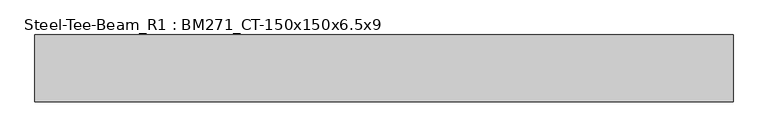
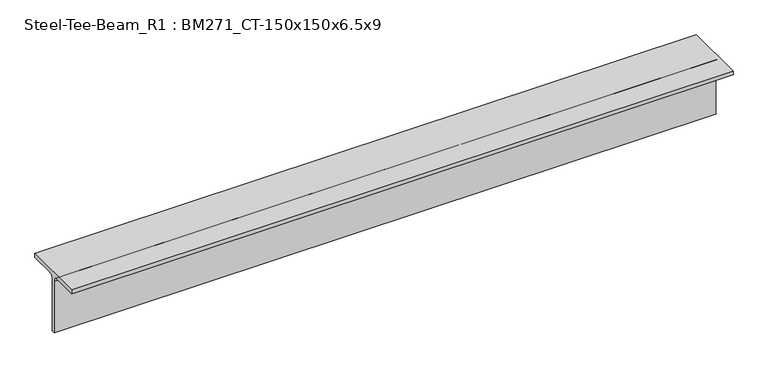
"""IFC4 building model written with IfcOpenShell, lengths in millimetres: member geometry, Steel-Tee-Beam_R1 : BM271_CT-150x150x6.5x9."""

from ifc_helpers import new_model, si_unit, point, frame, frame_2d, origin, place, context, project, spatial, polyline, circle_curve, trimmed, segment, composite_curve, outline, extrude, source, transform, mapped, element, save


def steel_tee_beam_r1_bm271_ct_150x150x6_5x9_cc699060(model_context):
    return source(origin(), model_context, "Body", "SweptSolid", [
        extrude(outline(composite_curve([segment(polyline([(-75.0, 75.0), (75.0, 75.0), (75.0, 66.0), (16.25, 66.0)]), True, "CONTINUOUS"), segment(trimmed(circle_curve(frame_2d((16.25, 53.0)), 13.0), [point((16.25, 66.0))], [point((3.25, 53.0))], True, "CARTESIAN"), True, "CONTINUOUS"), segment(polyline([(3.25, 53.0), (3.25, -75.0), (-3.25, -75.0), (-3.25, 53.0)]), True, "CONTINUOUS"), segment(trimmed(circle_curve(frame_2d((-16.25, 53.0)), 13.0), [point((-3.25, 53.0))], [point((-16.25, 66.0))], True, "CARTESIAN"), True, "CONTINUOUS"), segment(polyline([(-16.25, 66.0), (-75.0, 66.0), (-75.0, 75.0)]), True, "CONTINUOUS")], self_intersect=False)), frame((-860.2325267, 0.0, 0.0), z_axis=(1.0, 0.0, 0.0), x_axis=(0.0, 1.0, 0.0)), (0.0, 0.0, 1.0), 1562.0258541),
    ])


if __name__ == "__main__":
    model = new_model("IFC4")
    model_context = context("Model", 3, world=origin())
    ifc_project = project(units=[si_unit("LENGTHUNIT", "METRE", prefix="MILLI")], contexts=[model_context])
    site = spatial("IfcSite", under=ifc_project)
    building = spatial("IfcBuilding", under=site)
    placement = place(None, origin())
    steel_tee_beam_r1_bm271_ct_150x150x6_5x9_shape = steel_tee_beam_r1_bm271_ct_150x150x6_5x9_cc699060(model_context)
    element("IfcMember", 1, ObjectType="Steel-Tee-Beam_R1 : BM271_CT-150x150x6.5x9", at=placement, inside=building, context=model_context, shape_type="MappedRepresentation", body=[
        mapped(steel_tee_beam_r1_bm271_ct_150x150x6_5x9_shape, transform((0.0, 0.0, 0.0), x_axis=(1.0, 0.0, 0.0), y_axis=(0.0, 1.0, 0.0), z_axis=(0.0, 0.0, 1.0))),
    ])
    save(model, "model.ifc")

# Revit data of these elements
# Type "Steel-Tee-Beam_R1 : BM271_CT-150x150x6.5x9"
#   Keynote = "CT-150x150x6.5x9"
#   Surface Area = 0.588841 m²/m
#   Section Area = 23.3904 cm²
#   Mass per Unit Length = 18.3614 kg/m
#   Length [instance default] = 1.5240 m
#   bf = 0.1500 m
#   d = 0.1500 m
#   k = 0.0220 m
#   r = 0.0130 m
#   tf = 0.0090 m
#   tw = 0.0065 m
#   hec_material4 [instance default] = none
#   hec_material3 [instance default] = none
#   hec_material2 [instance default] = none
#   hec_material1 [instance default] = none
#   Structural Material [instance default] = Steel, 45-345
#   Assembly Code = ""
# Element 1 (IfcMember, "Steel-Tee-Beam_R1 : BM271_CT-150x150x6.5x9")
#   Structural Material = none
# Materials
#   "Steel, 45-345": class "Metal", colour RGB 189 187 185, transparency 0, Description = "Steel 345 MPa", Cost = 0
